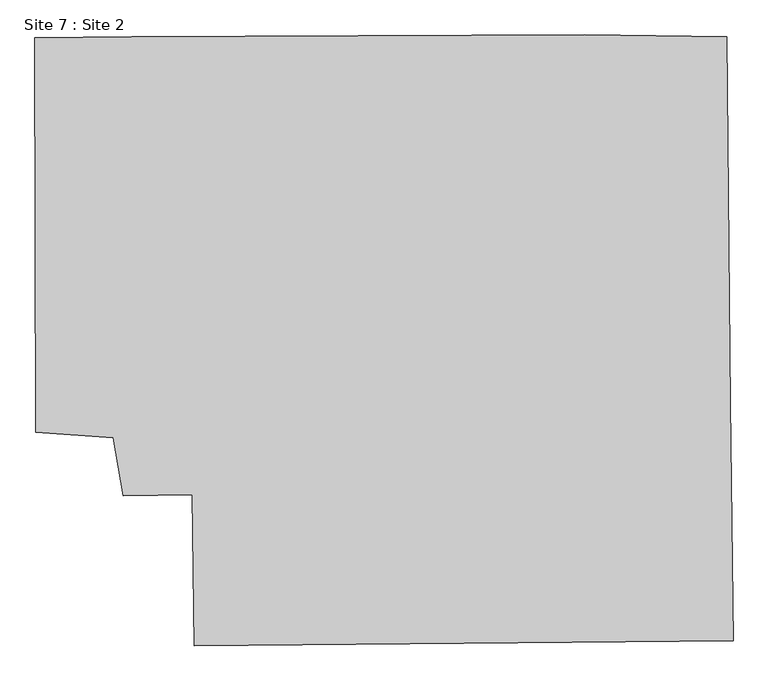
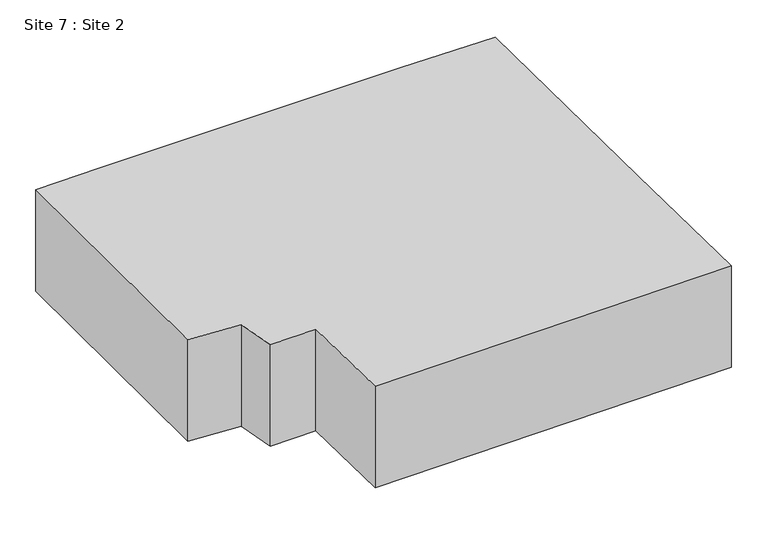
"""IFC4 building model written with IfcOpenShell, lengths in millimetres: geographic element geometry, Site 7 : Site 2."""

from ifc_helpers import new_model, si_unit, frame, origin, place, context, project, spatial, polyline, outline, extrude, source, transform, mapped, element, save


def site_7_site_2_ff44412e(model_context):
    return source(origin(), model_context, "Body", "SweptSolid", [
        extrude(outline(polyline([(-25965.0741058, 21462.89147), (-25822.1944366, 10283.8077133), (-51228.3606592, 10042.2224173), (-51328.5182912, 17156.3070396), (-54580.8499882, 17101.8159228), (-55049.0577043, 19852.0270273), (-58703.3306033, 20108.226609), (-58738.7748805, 38703.1705401), (-54165.78092, 38738.5288976), (-32826.1320487, 38835.809938), (-26121.2378387, 38738.6744849), (-25965.0741058, 21462.89147)])), frame((0.0, 0.0, 266395.2), z_axis=(0.0, 0.0, 1.0), x_axis=(1.0, 0.0, 0.0)), (0.0, 0.0, 1.0), 7620.0),
    ])


if __name__ == "__main__":
    model = new_model("IFC4")
    model_context = context("Model", 3, world=origin())
    ifc_project = project(units=[si_unit("LENGTHUNIT", "METRE", prefix="MILLI")], contexts=[model_context])
    site = spatial("IfcSite", under=ifc_project)
    building = spatial("IfcBuilding", under=site)
    placement = place(None, origin())
    site_7_site_2_shape = site_7_site_2_ff44412e(model_context)
    element("IfcGeographicElement", 1, ObjectType="Site 7 : Site 2", at=placement, inside=building, context=model_context, shape_type="MappedRepresentation", body=[
        mapped(site_7_site_2_shape, transform((0.0, 0.0, 0.0), x_axis=(1.0, 0.0, 0.0), y_axis=(0.0, 1.0, 0.0), z_axis=(0.0, 0.0, 1.0))),
    ])
    save(model, "model.ifc")

# Revit data of these elements
# Element 1 (IfcGeographicElement, "Site 7 : Site 2")
#   Materials on its faces: "EXISTING BUILDING"
# Materials
#   "EXISTING BUILDING": class "Generic", colour RGB 120 120 120, transparency 0, Cost = 0
